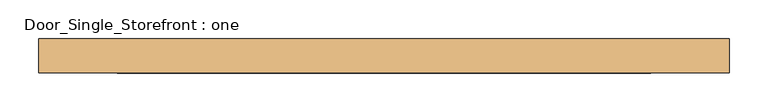
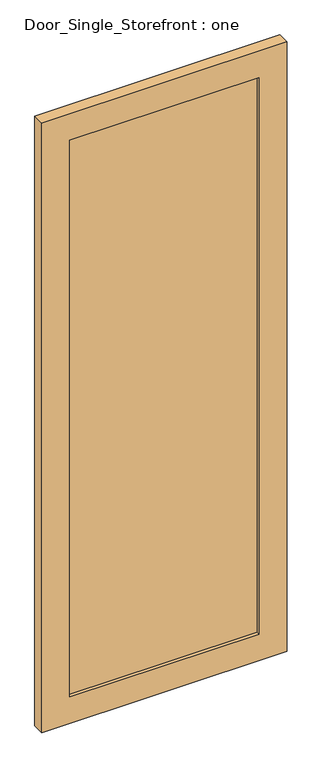
"""IFC4 building model written with IfcOpenShell, lengths in millimetres: door geometry, Door_Single_Storefront : one."""

from ifc_helpers import new_model, si_unit, frame, origin, place, context, project, spatial, polyline, outline, extrude, source, transform, mapped, element, save


def door_single_storefront_one_ff6ac5e0(model_context):
    return source(origin(), model_context, "Body", "SweptSolid", [
        extrude(outline(polyline([(2349.5, -446.88125), (0.0, -446.88125), (0.0, 446.88125), (2349.5, 446.88125), (2349.5, -446.88125)]), holes=[polyline([(101.6, 345.28125), (101.6, -345.28125), (2247.9, -345.28125), (2247.9, 345.28125), (101.6, 345.28125)])]), frame((0.0, -50.8, 0.0), z_axis=(0.0, 1.0, 0.0), x_axis=(0.0, 0.0, 1.0)), (0.0, 0.0, 1.0), 44.45),
        extrude(outline(polyline([(345.28125, -19.05), (345.28125, -38.1), (-345.28125, -38.1), (-345.28125, -19.05), (345.28125, -19.05)])), frame((0.0, 0.0, 101.6), z_axis=(0.0, 0.0, 1.0), x_axis=(1.0, 0.0, 0.0)), (0.0, 0.0, 1.0), 2146.3),
    ])


if __name__ == "__main__":
    model = new_model("IFC4")
    model_context = context("Model", 3, world=origin())
    ifc_project = project(units=[si_unit("LENGTHUNIT", "METRE", prefix="MILLI")], contexts=[model_context])
    site = spatial("IfcSite", under=ifc_project)
    building = spatial("IfcBuilding", under=site)
    placement = place(None, origin())
    door_single_storefront_one_shape = door_single_storefront_one_ff6ac5e0(model_context)
    element("IfcDoor", 1, ObjectType="Door_Single_Storefront : one", at=placement, inside=building, context=model_context, shape_type="MappedRepresentation", body=[
        mapped(door_single_storefront_one_shape, transform((0.0, 0.0, 0.0), x_axis=(1.0, 0.0, 0.0), y_axis=(0.0, 1.0, 0.0), z_axis=(0.0, 0.0, 1.0))),
    ])
    save(model, "model.ifc")

# Revit data of these elements
# Type "Door_Single_Storefront : one"
#   Type Mark = "27"
#   Analytic Construction = "<None>"
#   Stile_Width = 0' - 4"
#   Door_Thickness = 0' - 1 3/4"
#   Door_Offset = 0' - 2"
#   Glass_Material = Glass
#   Frame_Material = Aluminum
#   Function = (empty or 0)
# Element 1 (IfcDoor, "Door_Single_Storefront : one")
#   Materials on its faces: "Aluminum", "Glass"
# Materials
#   "Glass": class "Glass", colour RGB 0 128 192, transparency 0.75, Description = "Soda Lime Glass", Cost = 0
#   "Aluminum": class "Metal", colour RGB 247 247 247, transparency 0, Description = "Aluminum 6061", Cost = 0
